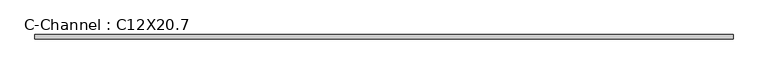
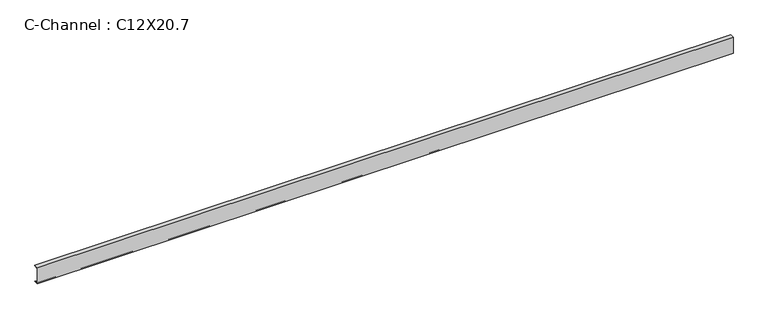
"""IFC4 building model written with IfcOpenShell, lengths in millimetres: beam geometry, C-Channel : C12X20.7."""

from ifc_helpers import new_model, si_unit, point, frame, frame_2d, origin, place, context, project, spatial, polyline, circle_curve, trimmed, segment, composite_curve, outline, extrude, source, transform, mapped, element, save


def c_channel_c12x20_7_89c3d779(model_context):
    return source(origin(), model_context, "Body", "SweptSolid", [
        extrude(outline(composite_curve([segment(polyline([(-17.7292, 152.4), (56.9468, 152.4)]), True, "CONTINUOUS"), segment(trimmed(circle_curve(frame_2d((44.2214, 152.4)), 12.7254), [point((56.9468, 152.4))], [point((44.2214, 139.6746))], False, "CARTESIAN"), True, "CONTINUOUS"), segment(polyline([(44.2214, 139.6746), (-10.5664, 130.997065), (-10.5664, -130.997065), (44.2214, -139.6746)]), True, "CONTINUOUS"), segment(trimmed(circle_curve(frame_2d((44.2214, -152.4)), 12.7254), [point((44.2214, -139.6746))], [point((56.9468, -152.4))], False, "CARTESIAN"), True, "CONTINUOUS"), segment(polyline([(56.9468, -152.4), (-17.7292, -152.4), (-17.7292, 152.4)]), True, "CONTINUOUS")], self_intersect=False)), frame((-6182.3330928, 0.0, 0.0), z_axis=(1.0, 0.0, 0.0), x_axis=(0.0, 1.0, 0.0)), (0.0, 0.0, 1.0), 12402.5284345),
    ])


if __name__ == "__main__":
    model = new_model("IFC4")
    model_context = context("Model", 3, world=origin())
    ifc_project = project(units=[si_unit("LENGTHUNIT", "METRE", prefix="MILLI")], contexts=[model_context])
    site = spatial("IfcSite", under=ifc_project)
    building = spatial("IfcBuilding", under=site)
    placement = place(None, origin())
    c_channel_c12x20_7_shape = c_channel_c12x20_7_89c3d779(model_context)
    element("IfcBeam", 1, ObjectType="C-Channel : C12X20.7", at=placement, inside=building, context=model_context, shape_type="MappedRepresentation", body=[
        mapped(c_channel_c12x20_7_shape, transform((0.0, 0.0, 0.0), x_axis=(1.0, 0.0, 0.0), y_axis=(0.0, 1.0, 0.0), z_axis=(0.0, 0.0, 1.0))),
    ])
    save(model, "model.ifc")

# Revit data of these elements
# Type "C-Channel : C12X20.7"
#   Assembly Code = "B10"
#   W = 20.7
#   Start Extension Calculation [instance default] = 10' - 0"
#   Start Extension [instance default] = -0' - 0 1/2"
#   End Extension Calculation [instance default] = 10' - 0"
#   End Extension [instance default] = -0' - 0 1/2"
#   Length [instance default] = 5' - 0"
#   bf = 0' - 2.94"
#   d = 1' - 0"
#   tf = 0' - 0.501"
#   tw = 0' - 0.282"
#   x = 0' - 0.698"
#   A = 0.0422222 SF
#   Structural Material [instance default] = Metal - Steel - ASTM A36
# Element 1 (IfcBeam, "C-Channel : C12X20.7")
#   Materials on its faces: "Metal - Steel - ASTM A36"
# Materials
#   "Metal - Steel - ASTM A36": class "Metal", colour RGB 199 199 199, transparency 0
